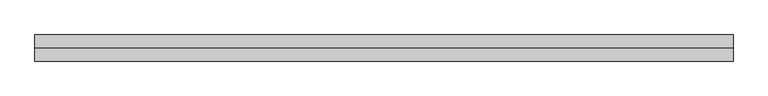
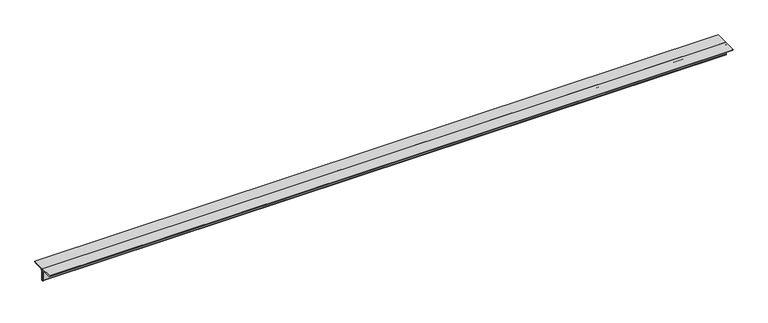
"""IFC4 building model written with IfcOpenShell, lengths in millimetres: member geometry, Steel Framing_2Ls_KS : H_SB_AR_S02_2Ls-100x100x10_VBR1."""

import ifcopenshell
import ifcopenshell.guid

model = None  # the IFC model being written
_history = None  # IfcOwnerHistory: only IFC2X3 demands one
_inside = {}  # id of a spatial element -> (the spatial element, [elements in it])
_under = {}  # id of a project, library or spatial element -> (it, [spatial elements below it])
_declared = {}  # id of a project -> (the project, [libraries it declares])
_typed = {}  # id of a type object -> (the type object, [elements of that type])
_made_of = {}  # id of a material, layer set ... -> (it, [elements and type objects made of it])


def new_model(schema):
    """Start an empty IFC model of exactly this schema.

    Asked for "IFC4X3", IfcOpenShell would pick the latest addendum, in which some entities
    have other attributes; the version numbers below select the first issue.
    IFC2X3 requires an IfcOwnerHistory on every rooted entity: one is made here for all.
    """
    global model, _history
    if schema == "IFC4X3":
        model = ifcopenshell.file(schema_version=(4, 3, 0, 0))
    else:
        model = ifcopenshell.file(schema=schema)
    _inside.clear()
    _under.clear()
    _declared.clear()
    _typed.clear()
    _made_of.clear()
    _history = None
    if model.schema == "IFC2X3":
        org = make("IfcOrganization", Name="unknown")
        user = make(
            "IfcPersonAndOrganization",
            ThePerson=make("IfcPerson", FamilyName="unknown"),
            TheOrganization=org,
        )
        app = make(
            "IfcApplication",
            ApplicationDeveloper=org,
            Version="unknown",
            ApplicationFullName="unknown",
            ApplicationIdentifier="unknown",
        )
        _history = make(
            "IfcOwnerHistory",
            OwningUser=user,
            OwningApplication=app,
            ChangeAction="ADDED",
            CreationDate=0,
        )
    return model


def make(cls, **values):
    """One entity of the class cls with the attributes given. An attribute that is None is left unset."""
    return model.create_entity(
        cls, **{name: value for name, value in values.items() if value is not None}
    )


def rooted(cls, **values):
    """An entity with a GlobalId (a new one), such as an element, a storey or a relation."""
    return make(cls, GlobalId=ifcopenshell.guid.new(), OwnerHistory=_history, **values)


def si_unit(unit_type, name, prefix=None):
    """IfcSIUnit, for example si_unit("LENGTHUNIT", "METRE", prefix="MILLI")."""
    return make("IfcSIUnit", UnitType=unit_type, Prefix=prefix, Name=name)


def assignment(units):
    """IfcUnitAssignment: the units of a project."""
    return None if units is None else make("IfcUnitAssignment", Units=units)


def point(xyz):
    """IfcCartesianPoint."""
    return None if xyz is None else make("IfcCartesianPoint", Coordinates=xyz)


def direction(xyz):
    """IfcDirection."""
    return None if xyz is None else make("IfcDirection", DirectionRatios=xyz)


def frame(location, z_axis=None, x_axis=None):
    """IfcAxis2Placement3D, a coordinate frame: its origin and axes. An axis left out is left unset."""
    return make(
        "IfcAxis2Placement3D",
        Location=point(location),
        Axis=direction(z_axis),
        RefDirection=direction(x_axis),
    )


def frame_2d(location, x_axis=None):
    """IfcAxis2Placement2D, a coordinate frame in the plane: its origin and x axis."""
    return make(
        "IfcAxis2Placement2D", Location=point(location), RefDirection=direction(x_axis)
    )


def origin():
    """The frame at (0, 0, 0) with its axes left unset."""
    return frame((0.0, 0.0, 0.0))


def place(relative_to, where):
    """IfcLocalPlacement: puts the frame where relative to a parent placement (None: the world)."""
    return make(
        "IfcLocalPlacement", PlacementRelTo=relative_to, RelativePlacement=where
    )


def context(
    kind, dimensions, precision=None, world=None, true_north=None, identifier=None
):
    """IfcGeometricRepresentationContext, for example the 3D "Model" context."""
    return make(
        "IfcGeometricRepresentationContext",
        ContextIdentifier=identifier,
        ContextType=kind,
        CoordinateSpaceDimension=dimensions,
        Precision=precision,
        WorldCoordinateSystem=world,
        TrueNorth=true_north,
    )


def project(units=None, contexts=None):
    """IfcProject with its units and contexts."""
    return rooted(
        "IfcProject",
        Name="project",
        RepresentationContexts=contexts,
        UnitsInContext=assignment(units),
    )


def spatial(cls, under=None, at=None, **own):
    """A site, building, storey or space (cls), placed at a placement, below another one or the project."""
    s = rooted(cls, ObjectPlacement=at, **own)
    if under is not None:
        _under.setdefault(under.id(), (under, []))[1].append(s)
    return s


def polyline(points):
    """IfcPolyline through the points."""
    return make("IfcPolyline", Points=[point(p) for p in points])


def circle_curve(where, radius):
    """IfcCircle in the frame where."""
    return make("IfcCircle", Position=where, Radius=radius)


def trimmed(basis, trim1, trim2, sense, master):
    """IfcTrimmedCurve: the piece of a basis curve between two trims."""
    return make(
        "IfcTrimmedCurve",
        BasisCurve=basis,
        Trim1=trim1,
        Trim2=trim2,
        SenseAgreement=sense,
        MasterRepresentation=master,
    )


def segment(curve, same_sense, transition):
    """IfcCompositeCurveSegment."""
    return make(
        "IfcCompositeCurveSegment",
        Transition=transition,
        SameSense=same_sense,
        ParentCurve=curve,
    )


def composite_curve(segments, self_intersect=None):
    """IfcCompositeCurve: segments joined end to end."""
    return make("IfcCompositeCurve", Segments=segments, SelfIntersect=self_intersect)


def outline(outer, holes=None, kind="AREA"):
    """IfcArbitraryClosedProfileDef: a profile drawn as a closed curve; with holes, ...WithVoids."""
    if holes is None:
        return make("IfcArbitraryClosedProfileDef", ProfileType=kind, OuterCurve=outer)
    return make(
        "IfcArbitraryProfileDefWithVoids",
        ProfileType=kind,
        OuterCurve=outer,
        InnerCurves=holes,
    )


def extrude(swept, where, along, depth):
    """IfcExtrudedAreaSolid: the profile swept, set in the frame where, extruded along a direction by depth."""
    return make(
        "IfcExtrudedAreaSolid",
        SweptArea=swept,
        Position=where,
        ExtrudedDirection=direction(along),
        Depth=depth,
    )


def shape(context_of_items, identifier, shape_type, items):
    """IfcShapeRepresentation: the items that make up one representation, for example the "Body"."""
    return make(
        "IfcShapeRepresentation",
        ContextOfItems=context_of_items,
        RepresentationIdentifier=identifier,
        RepresentationType=shape_type,
        Items=items,
    )


def source(mapping_origin, context_of_items, identifier, shape_type, items):
    """IfcRepresentationMap: a shape defined once, which mapped items show again and again."""
    return make(
        "IfcRepresentationMap",
        MappingOrigin=mapping_origin,
        MappedRepresentation=shape(context_of_items, identifier, shape_type, items),
    )


def transform(
    local_origin,
    x_axis=None,
    y_axis=None,
    z_axis=None,
    scale=None,
    scale2=None,
    scale3=None,
    uniform=True,
):
    """IfcCartesianTransformationOperator3D, or its non-uniform kind. x_axis, y_axis, z_axis: its Axis1, 2, 3."""
    if uniform:
        return make(
            "IfcCartesianTransformationOperator3D",
            Axis1=direction(x_axis),
            Axis2=direction(y_axis),
            LocalOrigin=point(local_origin),
            Scale=scale,
            Axis3=direction(z_axis),
        )
    return make(
        "IfcCartesianTransformationOperator3DnonUniform",
        Axis1=direction(x_axis),
        Axis2=direction(y_axis),
        LocalOrigin=point(local_origin),
        Scale=scale,
        Axis3=direction(z_axis),
        Scale2=scale2,
        Scale3=scale3,
    )


def mapped(mapping_source, mapping_target):
    """IfcMappedItem: shows the shape of a source again, moved by a transform."""
    return make(
        "IfcMappedItem", MappingSource=mapping_source, MappingTarget=mapping_target
    )


def made_of(thing, what):
    """Note that an element or type object is made of a material, layer set ...; save() writes the relation."""
    if what is not None:
        _made_of.setdefault(what.id(), (what, []))[1].append(thing)
    return thing


def element(
    cls,
    number,
    at=None,
    inside=None,
    cuts=None,
    type_object=None,
    material=None,
    context=None,
    identifier="Body",
    shape_type=None,
    held_by="IfcProductDefinitionShape",
    body=None,
    shapes=None,
    **own,
):
    """One element of the class cls, such as IfcWall. Its Tag is "e" and its number.

    at: its placement. inside: the storey or other place that contains it. cuts: it is an
    opening in that element (IfcRelVoidsElement). A single representation is given by context,
    identifier, shape_type and body (its items); several are given by shapes. held_by: the class
    of the entity that holds the representations. save() writes the other relations.
    """
    e = rooted(cls, Tag="e%d" % number, ObjectPlacement=at, **own)
    if body is not None:
        shapes = [shape(context, identifier, shape_type, body)]
    if shapes is not None:
        e.Representation = make(held_by, Representations=shapes)
    if inside is not None:
        _inside.setdefault(inside.id(), (inside, []))[1].append(e)
    if cuts is not None:
        rooted(
            "IfcRelVoidsElement", RelatingBuildingElement=cuts, RelatedOpeningElement=e
        )
    if type_object is not None:
        _typed.setdefault(type_object.id(), (type_object, []))[1].append(e)
    return made_of(e, material)


def aggregate(whole, parts):
    """IfcRelAggregates: a whole, such as a stair, and the parts it consists of."""
    return rooted("IfcRelAggregates", RelatingObject=whole, RelatedObjects=parts)


def save(model, path):
    """Write the relations noted so far, then the file.

    IfcRelAggregates (storeys below a building ...), IfcRelContainedInSpatialStructure (elements
    in a storey), IfcRelDefinesByType, IfcRelAssociatesMaterial and IfcRelDeclares: one each for
    every whole, place, type object, material and project.
    """
    for whole, parts in _under.values():
        aggregate(whole, parts)
    for where, things in _inside.values():
        rooted(
            "IfcRelContainedInSpatialStructure",
            RelatedElements=things,
            RelatingStructure=where,
        )
    for kind, things in _typed.values():
        rooted("IfcRelDefinesByType", RelatedObjects=things, RelatingType=kind)
    for what, things in _made_of.values():
        rooted("IfcRelAssociatesMaterial", RelatedObjects=things, RelatingMaterial=what)
    for by, libraries in _declared.values():
        rooted("IfcRelDeclares", RelatingContext=by, RelatedDefinitions=libraries)
    model.write(path)


def member_5d471435(model_context):
    return source(origin(), model_context, "Body", "SweptSolid", [
        extrude(outline(composite_curve([segment(polyline([(0.0, 28.2), (100.0, 28.2)]), True, "CONTINUOUS"), segment(trimmed(circle_curve(frame_2d((90.0, 28.2)), 10.0), [point((100.0, 28.2))], [point((90.0, 18.2))], False, "CARTESIAN"), True, "CONTINUOUS"), segment(polyline([(90.0, 18.2), (20.0, 18.2)]), True, "CONTINUOUS"), segment(trimmed(circle_curve(frame_2d((20.0, 8.2)), 10.0), [point((20.0, 18.2))], [point((10.0, 8.2))], True, "CARTESIAN"), True, "CONTINUOUS"), segment(polyline([(10.0, 8.2), (10.0, -61.8)]), True, "CONTINUOUS"), segment(trimmed(circle_curve(frame_2d((0.0, -61.8)), 10.0), [point((10.0, -61.8))], [point((0.0, -71.8))], False, "CARTESIAN"), True, "CONTINUOUS"), segment(polyline([(0.0, -71.8), (0.0, 28.2)]), True, "CONTINUOUS")], self_intersect=False)), frame((-2755.311669, 0.0, 0.0), z_axis=(1.0, 0.0, 0.0), x_axis=(0.0, 1.0, 0.0)), (0.0, 0.0, 1.0), 5345.6471524),
        extrude(outline(composite_curve([segment(polyline([(0.0, 28.2), (0.0, -71.8)]), True, "CONTINUOUS"), segment(trimmed(circle_curve(frame_2d((0.0, -61.8)), 10.0), [point((0.0, -71.8))], [point((-10.0, -61.8))], False, "CARTESIAN"), True, "CONTINUOUS"), segment(polyline([(-10.0, -61.8), (-10.0, 8.2)]), True, "CONTINUOUS"), segment(trimmed(circle_curve(frame_2d((-20.0, 8.2)), 10.0), [point((-10.0, 8.2))], [point((-20.0, 18.2))], True, "CARTESIAN"), True, "CONTINUOUS"), segment(polyline([(-20.0, 18.2), (-90.0, 18.2)]), True, "CONTINUOUS"), segment(trimmed(circle_curve(frame_2d((-90.0, 28.2)), 10.0), [point((-90.0, 18.2))], [point((-100.0, 28.2))], False, "CARTESIAN"), True, "CONTINUOUS"), segment(polyline([(-100.0, 28.2), (0.0, 28.2)]), True, "CONTINUOUS")], self_intersect=False)), frame((-2755.311669, 0.0, 0.0), z_axis=(1.0, 0.0, 0.0), x_axis=(0.0, 1.0, 0.0)), (0.0, 0.0, 1.0), 5345.6471524),
    ])


if __name__ == "__main__":
    model = new_model("IFC4")
    model_context = context("Model", 3, world=origin())
    ifc_project = project(units=[si_unit("LENGTHUNIT", "METRE", prefix="MILLI")], contexts=[model_context])
    site = spatial("IfcSite", under=ifc_project)
    building = spatial("IfcBuilding", under=site)
    placement = place(None, origin())
    member_shape = member_5d471435(model_context)
    element("IfcMember", 1, ObjectType="Steel Framing_2Ls_KS : H_SB_AR_S02_2Ls-100x100x10_VBR1", at=placement, inside=building, context=model_context, shape_type="MappedRepresentation", body=[
        mapped(member_shape, transform((0.0, 0.0, 0.0), x_axis=(1.0, 0.0, 0.0), y_axis=(0.0, 1.0, 0.0), z_axis=(0.0, 0.0, 1.0))),
    ])
    save(model, "model.ifc")

# Revit data of these elements
# Type "Steel Framing_2Ls_KS : H_SB_AR_S02_2Ls-100x100x10_VBR1"
#   Type Comments = "MAIN"
#   Type Mark = "VBR1"
#   H_SectionID = "2Ls-100x100x10"
#   Assembly Code = "B10"
#   Legs = "LLBB"
#   H_Ratio for Additional Steel Plate = 0.2
#   W = 0
#   Perimeter = 0.80 m²/m
#   Nominal Weight = 29.80 kgf/m
#   Length [instance default] = 1524 mm
#   Space = 0 mm
#   b = 100 mm
#   d = 100 mm
#   t = 10 mm
#   y = 28.2 mm
#   A = 0.0038 m²
#   Structural Material [instance default] = Steel, 45-345
# Element 1 (IfcMember, "Steel Framing_2Ls_KS : H_SB_AR_S02_2Ls-100x100x10_VBR1")
#   Materials on its faces: "Steel, 45-345"
# Materials
#   "Steel, 45-345": class "Metal", colour RGB 189 187 185, transparency 0, Description = "Steel 345 MPa", Cost = 0
